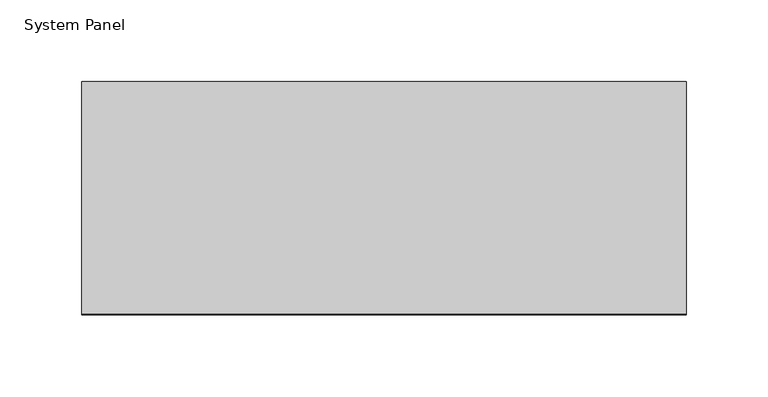
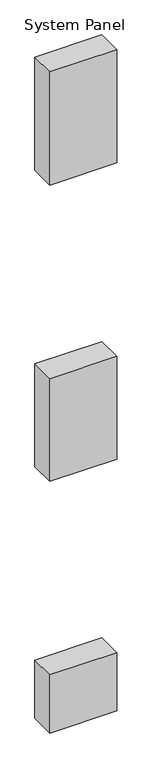
"""IFC4 building model written with IfcOpenShell, lengths in millimetres: plate geometry, System Panel : NLRS_21_CWP_hsb-vulling minerale wol 142 _gen_rsf."""

from ifc_helpers import new_model, si_unit, frame, origin, origin_with_axes, place, context, project, spatial, polyline, outline, extrude, source, transform, mapped, element, save


def system_panel_bba4faf4(model_context):
    return source(origin(), model_context, "Body", "SweptSolid", [
        extrude(outline(polyline([(184.5, -71.0), (-184.5, -71.0), (-184.5, 71.0), (184.5, 71.0), (184.5, -71.0)])), frame((0.0, 0.0, 3190.0), z_axis=(0.0, 0.0, 1.0), x_axis=(1.0, 0.0, 0.0)), (0.0, 0.0, 1.0), 659.0),
        extrude(outline(polyline([(184.5, -71.0), (-184.5, -71.0), (-184.5, 71.0), (184.5, 71.0), (184.5, -71.0)])), frame((0.0, 0.0, 1465.0), z_axis=(0.0, 0.0, 1.0), x_axis=(1.0, 0.0, 0.0)), (0.0, 0.0, 1.0), 599.0),
        extrude(outline(polyline([(184.5, -71.0), (-184.5, -71.0), (-184.5, 71.0), (184.5, 71.0), (184.5, -71.0)])), origin_with_axes(), (0.0, 0.0, 1.0), 339.0),
    ])


if __name__ == "__main__":
    model = new_model("IFC4")
    model_context = context("Model", 3, world=origin())
    ifc_project = project(units=[si_unit("LENGTHUNIT", "METRE", prefix="MILLI")], contexts=[model_context])
    site = spatial("IfcSite", under=ifc_project)
    building = spatial("IfcBuilding", under=site)
    placement = place(None, origin())
    system_panel_shape = system_panel_bba4faf4(model_context)
    element("IfcPlate", 1, ObjectType="System Panel : NLRS_21_CWP_hsb-vulling minerale wol 142 _gen_rsf", at=placement, inside=building, context=model_context, shape_type="MappedRepresentation", body=[
        mapped(system_panel_shape, transform((0.0, 0.0, 0.0), x_axis=(1.0, 0.0, 0.0), y_axis=(0.0, 1.0, 0.0), z_axis=(0.0, 0.0, 1.0))),
    ])
    save(model, "model.ifc")

# Revit data of these elements
# Type "System Panel : NLRS_21_CWP_hsb-vulling minerale wol 142 _gen_rsf"
#   Export Type to IFC As = "IfcWall"
#   Type IfcGUID = "07M7mRoiH1CR8m_RSKIwpC"
#   Assembly Code = "21.23"
# Element 1 (IfcPlate, "System Panel : NLRS_21_CWP_hsb-vulling minerale wol 142 _gen_rsf")
#   Materials on its faces: "NLRS_m1_isolatie minerale wol_gen_rsf"
# Materials
#   "NLRS_m1_isolatie minerale wol_gen_rsf": class "M - Anorganische materialen", colour RGB 200 200 140, transparency 0, Keynote = "m1", Manufacturer = "Revit Standards Foundation", URL = "www.revitstandards.org", Description = "isolatie minerale wol", Cost = 0
